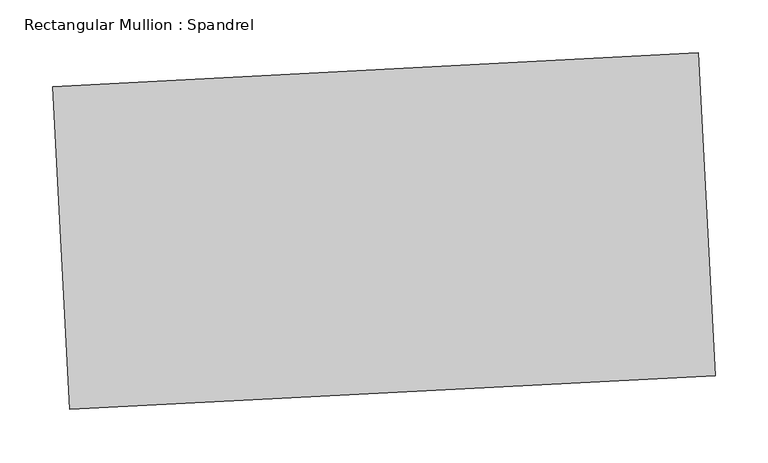
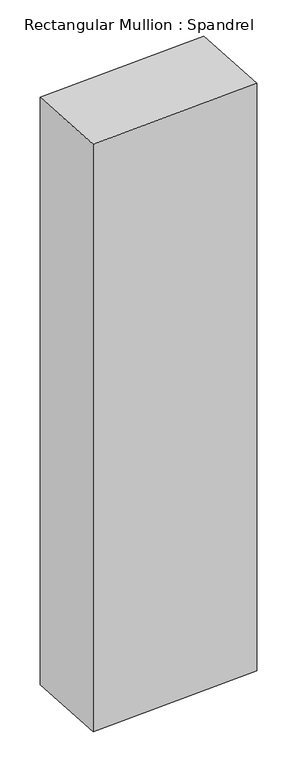
"""IFC4 building model written with IfcOpenShell, lengths in millimetres: member geometry, Rectangular Mullion : Spandrel."""

import ifcopenshell
import ifcopenshell.guid

model = None  # the IFC model being written
_history = None  # IfcOwnerHistory: only IFC2X3 demands one
_inside = {}  # id of a spatial element -> (the spatial element, [elements in it])
_under = {}  # id of a project, library or spatial element -> (it, [spatial elements below it])
_declared = {}  # id of a project -> (the project, [libraries it declares])
_typed = {}  # id of a type object -> (the type object, [elements of that type])
_made_of = {}  # id of a material, layer set ... -> (it, [elements and type objects made of it])


def new_model(schema):
    """Start an empty IFC model of exactly this schema.

    Asked for "IFC4X3", IfcOpenShell would pick the latest addendum, in which some entities
    have other attributes; the version numbers below select the first issue.
    IFC2X3 requires an IfcOwnerHistory on every rooted entity: one is made here for all.
    """
    global model, _history
    if schema == "IFC4X3":
        model = ifcopenshell.file(schema_version=(4, 3, 0, 0))
    else:
        model = ifcopenshell.file(schema=schema)
    _inside.clear()
    _under.clear()
    _declared.clear()
    _typed.clear()
    _made_of.clear()
    _history = None
    if model.schema == "IFC2X3":
        org = make("IfcOrganization", Name="unknown")
        user = make(
            "IfcPersonAndOrganization",
            ThePerson=make("IfcPerson", FamilyName="unknown"),
            TheOrganization=org,
        )
        app = make(
            "IfcApplication",
            ApplicationDeveloper=org,
            Version="unknown",
            ApplicationFullName="unknown",
            ApplicationIdentifier="unknown",
        )
        _history = make(
            "IfcOwnerHistory",
            OwningUser=user,
            OwningApplication=app,
            ChangeAction="ADDED",
            CreationDate=0,
        )
    return model


def make(cls, **values):
    """One entity of the class cls with the attributes given. An attribute that is None is left unset."""
    return model.create_entity(
        cls, **{name: value for name, value in values.items() if value is not None}
    )


def rooted(cls, **values):
    """An entity with a GlobalId (a new one), such as an element, a storey or a relation."""
    return make(cls, GlobalId=ifcopenshell.guid.new(), OwnerHistory=_history, **values)


def si_unit(unit_type, name, prefix=None):
    """IfcSIUnit, for example si_unit("LENGTHUNIT", "METRE", prefix="MILLI")."""
    return make("IfcSIUnit", UnitType=unit_type, Prefix=prefix, Name=name)


def assignment(units):
    """IfcUnitAssignment: the units of a project."""
    return None if units is None else make("IfcUnitAssignment", Units=units)


def point(xyz):
    """IfcCartesianPoint."""
    return None if xyz is None else make("IfcCartesianPoint", Coordinates=xyz)


def direction(xyz):
    """IfcDirection."""
    return None if xyz is None else make("IfcDirection", DirectionRatios=xyz)


def frame(location, z_axis=None, x_axis=None):
    """IfcAxis2Placement3D, a coordinate frame: its origin and axes. An axis left out is left unset."""
    return make(
        "IfcAxis2Placement3D",
        Location=point(location),
        Axis=direction(z_axis),
        RefDirection=direction(x_axis),
    )


def origin():
    """The frame at (0, 0, 0) with its axes left unset."""
    return frame((0.0, 0.0, 0.0))


def place(relative_to, where):
    """IfcLocalPlacement: puts the frame where relative to a parent placement (None: the world)."""
    return make(
        "IfcLocalPlacement", PlacementRelTo=relative_to, RelativePlacement=where
    )


def context(
    kind, dimensions, precision=None, world=None, true_north=None, identifier=None
):
    """IfcGeometricRepresentationContext, for example the 3D "Model" context."""
    return make(
        "IfcGeometricRepresentationContext",
        ContextIdentifier=identifier,
        ContextType=kind,
        CoordinateSpaceDimension=dimensions,
        Precision=precision,
        WorldCoordinateSystem=world,
        TrueNorth=true_north,
    )


def project(units=None, contexts=None):
    """IfcProject with its units and contexts."""
    return rooted(
        "IfcProject",
        Name="project",
        RepresentationContexts=contexts,
        UnitsInContext=assignment(units),
    )


def spatial(cls, under=None, at=None, **own):
    """A site, building, storey or space (cls), placed at a placement, below another one or the project."""
    s = rooted(cls, ObjectPlacement=at, **own)
    if under is not None:
        _under.setdefault(under.id(), (under, []))[1].append(s)
    return s


def polyline(points):
    """IfcPolyline through the points."""
    return make("IfcPolyline", Points=[point(p) for p in points])


def outline(outer, holes=None, kind="AREA"):
    """IfcArbitraryClosedProfileDef: a profile drawn as a closed curve; with holes, ...WithVoids."""
    if holes is None:
        return make("IfcArbitraryClosedProfileDef", ProfileType=kind, OuterCurve=outer)
    return make(
        "IfcArbitraryProfileDefWithVoids",
        ProfileType=kind,
        OuterCurve=outer,
        InnerCurves=holes,
    )


def extrude(swept, where, along, depth):
    """IfcExtrudedAreaSolid: the profile swept, set in the frame where, extruded along a direction by depth."""
    return make(
        "IfcExtrudedAreaSolid",
        SweptArea=swept,
        Position=where,
        ExtrudedDirection=direction(along),
        Depth=depth,
    )


def shape(context_of_items, identifier, shape_type, items):
    """IfcShapeRepresentation: the items that make up one representation, for example the "Body"."""
    return make(
        "IfcShapeRepresentation",
        ContextOfItems=context_of_items,
        RepresentationIdentifier=identifier,
        RepresentationType=shape_type,
        Items=items,
    )


def source(mapping_origin, context_of_items, identifier, shape_type, items):
    """IfcRepresentationMap: a shape defined once, which mapped items show again and again."""
    return make(
        "IfcRepresentationMap",
        MappingOrigin=mapping_origin,
        MappedRepresentation=shape(context_of_items, identifier, shape_type, items),
    )


def transform(
    local_origin,
    x_axis=None,
    y_axis=None,
    z_axis=None,
    scale=None,
    scale2=None,
    scale3=None,
    uniform=True,
):
    """IfcCartesianTransformationOperator3D, or its non-uniform kind. x_axis, y_axis, z_axis: its Axis1, 2, 3."""
    if uniform:
        return make(
            "IfcCartesianTransformationOperator3D",
            Axis1=direction(x_axis),
            Axis2=direction(y_axis),
            LocalOrigin=point(local_origin),
            Scale=scale,
            Axis3=direction(z_axis),
        )
    return make(
        "IfcCartesianTransformationOperator3DnonUniform",
        Axis1=direction(x_axis),
        Axis2=direction(y_axis),
        LocalOrigin=point(local_origin),
        Scale=scale,
        Axis3=direction(z_axis),
        Scale2=scale2,
        Scale3=scale3,
    )


def mapped(mapping_source, mapping_target):
    """IfcMappedItem: shows the shape of a source again, moved by a transform."""
    return make(
        "IfcMappedItem", MappingSource=mapping_source, MappingTarget=mapping_target
    )


def made_of(thing, what):
    """Note that an element or type object is made of a material, layer set ...; save() writes the relation."""
    if what is not None:
        _made_of.setdefault(what.id(), (what, []))[1].append(thing)
    return thing


def element(
    cls,
    number,
    at=None,
    inside=None,
    cuts=None,
    type_object=None,
    material=None,
    context=None,
    identifier="Body",
    shape_type=None,
    held_by="IfcProductDefinitionShape",
    body=None,
    shapes=None,
    **own,
):
    """One element of the class cls, such as IfcWall. Its Tag is "e" and its number.

    at: its placement. inside: the storey or other place that contains it. cuts: it is an
    opening in that element (IfcRelVoidsElement). A single representation is given by context,
    identifier, shape_type and body (its items); several are given by shapes. held_by: the class
    of the entity that holds the representations. save() writes the other relations.
    """
    e = rooted(cls, Tag="e%d" % number, ObjectPlacement=at, **own)
    if body is not None:
        shapes = [shape(context, identifier, shape_type, body)]
    if shapes is not None:
        e.Representation = make(held_by, Representations=shapes)
    if inside is not None:
        _inside.setdefault(inside.id(), (inside, []))[1].append(e)
    if cuts is not None:
        rooted(
            "IfcRelVoidsElement", RelatingBuildingElement=cuts, RelatedOpeningElement=e
        )
    if type_object is not None:
        _typed.setdefault(type_object.id(), (type_object, []))[1].append(e)
    return made_of(e, material)


def aggregate(whole, parts):
    """IfcRelAggregates: a whole, such as a stair, and the parts it consists of."""
    return rooted("IfcRelAggregates", RelatingObject=whole, RelatedObjects=parts)


def save(model, path):
    """Write the relations noted so far, then the file.

    IfcRelAggregates (storeys below a building ...), IfcRelContainedInSpatialStructure (elements
    in a storey), IfcRelDefinesByType, IfcRelAssociatesMaterial and IfcRelDeclares: one each for
    every whole, place, type object, material and project.
    """
    for whole, parts in _under.values():
        aggregate(whole, parts)
    for where, things in _inside.values():
        rooted(
            "IfcRelContainedInSpatialStructure",
            RelatedElements=things,
            RelatingStructure=where,
        )
    for kind, things in _typed.values():
        rooted("IfcRelDefinesByType", RelatedObjects=things, RelatingType=kind)
    for what, things in _made_of.values():
        rooted("IfcRelAssociatesMaterial", RelatedObjects=things, RelatingMaterial=what)
    for by, libraries in _declared.values():
        rooted("IfcRelDeclares", RelatingContext=by, RelatedDefinitions=libraries)
    model.write(path)


def rectangular_mullion_spandrel_dc5cde31(model_context):
    return source(origin(), model_context, "Body", "SweptSolid", [
        extrude(outline(polyline([(-617.1582819, 136.2391416), (-8.3937175, 168.1431406), (7.5582819, -136.2391416), (-601.2062825, -168.1431406), (-617.1582819, 136.2391416)])), frame((0.0, 0.0, -2238.2848233), z_axis=(0.0, 0.0, 1.0), x_axis=(1.0, 0.0, 0.0)), (0.0, 0.0, 1.0), 2238.2848233),
    ])


if __name__ == "__main__":
    model = new_model("IFC4")
    model_context = context("Model", 3, world=origin())
    ifc_project = project(units=[si_unit("LENGTHUNIT", "METRE", prefix="MILLI")], contexts=[model_context])
    site = spatial("IfcSite", under=ifc_project)
    building = spatial("IfcBuilding", under=site)
    placement = place(None, origin())
    rectangular_mullion_spandrel_shape = rectangular_mullion_spandrel_dc5cde31(model_context)
    element("IfcMember", 1, ObjectType="Rectangular Mullion : Spandrel", at=placement, inside=building, context=model_context, shape_type="MappedRepresentation", body=[
        mapped(rectangular_mullion_spandrel_shape, transform((0.0, 0.0, 0.0), x_axis=(1.0, 0.0, 0.0), y_axis=(0.0, 1.0, 0.0), z_axis=(0.0, 0.0, 1.0))),
    ])
    save(model, "model.ifc")

# Revit data of these elements
# Type "Rectangular Mullion : Spandrel"
#   built-in parameter 1007304 = 1 (stored number, unit not read)
#   built-in parameter 1007301 = 1 (stored number, unit not read)
#   built-in parameter 1007300 = 1 (stored number, unit not read)
# Element 1 (IfcMember, "Rectangular Mullion : Spandrel")
#   Materials on its faces: "Aluminum"
# Materials
#   "Aluminum": class "Metal", colour RGB 247 247 247, transparency 0, Description = "Aluminum 6061", Cost = 0
